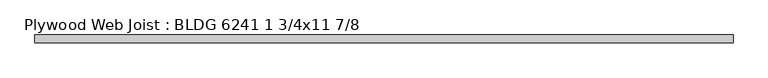
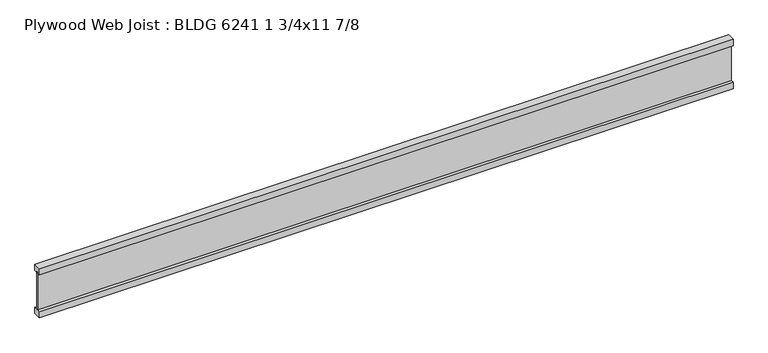
"""IFC4 building model written with IfcOpenShell, lengths in millimetres: beam geometry, Plywood Web Joist : BLDG 6241 1 3/4x11 7/8."""

from ifc_helpers import new_model, si_unit, frame, origin, place, context, project, spatial, polyline, outline, extrude, source, transform, mapped, element, save


def plywood_web_joist_bldg_6241_1_3_4x11_7_8_0dc58311(model_context):
    return source(origin(), model_context, "Body", "SweptSolid", [
        extrude(outline(polyline([(-22.225, 150.8125), (22.225, 150.8125), (22.225, 112.7125), (4.7625, 112.7125), (4.7625, 119.0625), (-4.7625, 119.0625), (-4.7625, 112.7125), (-22.225, 112.7125), (-22.225, 150.8125)])), frame((-2030.1401281, 0.0, 0.0), z_axis=(1.0, 0.0, 0.0), x_axis=(0.0, 1.0, 0.0)), (0.0, 0.0, 1.0), 4019.6434633),
        extrude(outline(polyline([(22.225, -112.7125), (22.225, -150.8125), (-22.225, -150.8125), (-22.225, -112.7125), (-4.7625, -112.7125), (-4.7625, -118.3285374), (4.7625, -118.3285374), (4.7625, -112.7125), (22.225, -112.7125)])), frame((-2030.1401281, 0.0, 0.0), z_axis=(1.0, 0.0, 0.0), x_axis=(0.0, 1.0, 0.0)), (0.0, 0.0, 1.0), 4019.6434633),
        extrude(outline(polyline([(1989.5033352, 4.7625), (1989.5033352, -4.7625), (-2030.1401281, -4.7625), (-2030.1401281, 4.7625), (1989.5033352, 4.7625)])), frame((0.0, 0.0, -118.3285374), z_axis=(0.0, 0.0, 1.0), x_axis=(1.0, 0.0, 0.0)), (0.0, 0.0, 1.0), 237.3910374),
    ])


if __name__ == "__main__":
    model = new_model("IFC4")
    model_context = context("Model", 3, world=origin())
    ifc_project = project(units=[si_unit("LENGTHUNIT", "METRE", prefix="MILLI")], contexts=[model_context])
    site = spatial("IfcSite", under=ifc_project)
    building = spatial("IfcBuilding", under=site)
    placement = place(None, origin())
    plywood_web_joist_bldg_6241_1_3_4x11_7_8_shape = plywood_web_joist_bldg_6241_1_3_4x11_7_8_0dc58311(model_context)
    element("IfcBeam", 1, ObjectType="Plywood Web Joist : BLDG 6241 1 3/4x11 7/8", at=placement, inside=building, context=model_context, shape_type="MappedRepresentation", body=[
        mapped(plywood_web_joist_bldg_6241_1_3_4x11_7_8_shape, transform((0.0, 0.0, 0.0), x_axis=(1.0, 0.0, 0.0), y_axis=(0.0, 1.0, 0.0), z_axis=(0.0, 0.0, 1.0))),
    ])
    save(model, "model.ifc")

# Revit data of these elements
# Type "Plywood Web Joist : BLDG 6241 1 3/4x11 7/8"
#   Assembly Code = "B10"
#   Length [instance default] = 5' - 0"
#   b = 0' - 1 3/4"
#   d = 0' - 11 7/8"
#   Structural Material [instance default] = Softwood, Lumber
# Element 1 (IfcBeam, "Plywood Web Joist : BLDG 6241 1 3/4x11 7/8")
#   Materials on its faces: "Softwood, Lumber"
# Materials
#   "Softwood, Lumber": class "Wood", colour RGB 223 192 134, transparency 0, Description = "Pinus Echinata", Cost = 0
